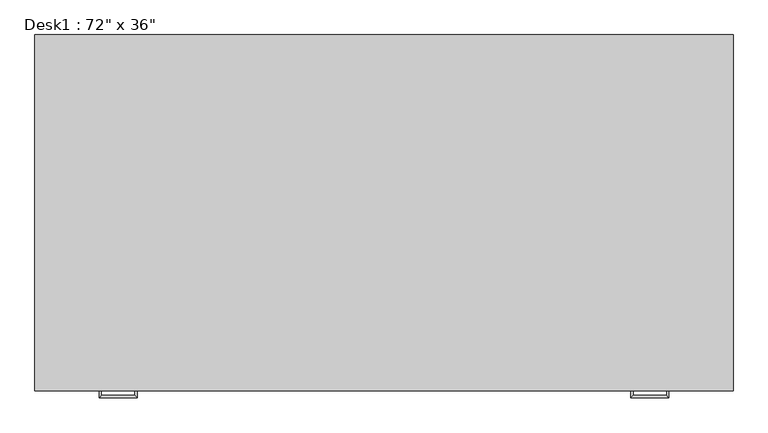
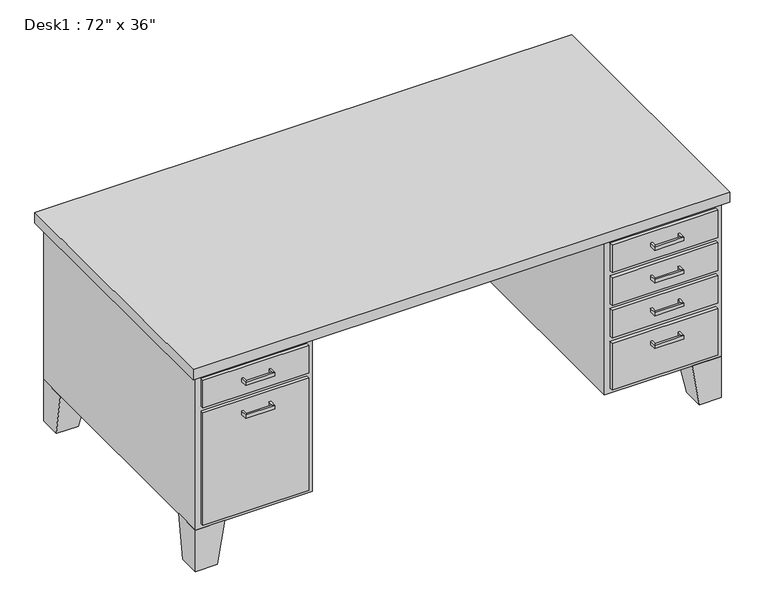
"""IFC4 building model written with IfcOpenShell, lengths in millimetres: furniture geometry."""

from ifc_helpers import new_model, si_unit, frame, origin, place, context, project, spatial, polyline, outline, extrude, faceted_brep, source, transform, mapped, element, save


def furniture_95783df2(model_context):
    return source(origin(), model_context, "Body", "SolidModel", [
        extrude(outline(polyline([(-133.35, -76.2), (234.95, -76.2), (234.95, -88.9), (-133.35, -88.9), (-133.35, -76.2)])), frame((0.0, 0.0, 603.25), z_axis=(0.0, 0.0, 1.0), x_axis=(1.0, 0.0, 0.0)), (0.0, 0.0, 1.0), 101.6),
        extrude(outline(polyline([(-133.35, -76.2), (234.95, -76.2), (234.95, -88.9), (-133.35, -88.9), (-133.35, -76.2)])), frame((0.0, 0.0, 171.45), z_axis=(0.0, 0.0, 1.0), x_axis=(1.0, 0.0, 0.0)), (0.0, 0.0, 1.0), 412.75),
        extrude(outline(polyline([(1289.05, -76.2), (1657.35, -76.2), (1657.35, -88.9), (1289.05, -88.9), (1289.05, -76.2)])), frame((0.0, 0.0, 603.25), z_axis=(0.0, 0.0, 1.0), x_axis=(1.0, 0.0, 0.0)), (0.0, 0.0, 1.0), 101.6),
        extrude(outline(polyline([(1289.05, -76.2), (1657.35, -76.2), (1657.35, -88.9), (1289.05, -88.9), (1289.05, -76.2)])), frame((0.0, 0.0, 171.45), z_axis=(0.0, 0.0, 1.0), x_axis=(1.0, 0.0, 0.0)), (0.0, 0.0, 1.0), 171.45),
        extrude(outline(polyline([(1289.05, -76.2), (1657.35, -76.2), (1657.35, -88.9), (1289.05, -88.9), (1289.05, -76.2)])), frame((0.0, 0.0, 482.6), z_axis=(0.0, 0.0, 1.0), x_axis=(1.0, 0.0, 0.0)), (0.0, 0.0, 1.0), 101.6),
        extrude(outline(polyline([(1289.05, -76.2), (1657.35, -76.2), (1657.35, -88.9), (1289.05, -88.9), (1289.05, -76.2)])), frame((0.0, 0.0, 361.95), z_axis=(0.0, 0.0, 1.0), x_axis=(1.0, 0.0, 0.0)), (0.0, 0.0, 1.0), 101.6),
        faceted_brep([(-50.8, -76.2, 152.4), (-50.8, 25.4, 152.4), (-152.4, 25.4, 152.4), (-152.4, -76.2, 152.4), (-76.2, -76.2, 0.0), (-152.4, -76.2, 0.0), (-152.4, 0.0, 0.0), (-76.2, 0.0, 0.0)], [[[0, 1, 2, 3]], [[4, 5, 6, 7]], [[4, 7, 1, 0]], [[7, 6, 2, 1]], [[6, 5, 3, 2]], [[5, 4, 0, 3]]]),
        faceted_brep([(-50.8, 838.2, 152.4), (-152.4, 838.2, 152.4), (-152.4, 736.6, 152.4), (-50.8, 736.6, 152.4), (-76.2, 838.2, 0.0), (-76.2, 762.0, 0.0), (-152.4, 762.0, 0.0), (-152.4, 838.2, 0.0)], [[[0, 1, 2, 3]], [[4, 5, 6, 7]], [[4, 7, 1, 0]], [[7, 6, 2, 1]], [[6, 5, 3, 2]], [[5, 4, 0, 3]]]),
        faceted_brep([(1574.8, 838.2, 152.4), (1574.8, 736.6, 152.4), (1676.4, 736.6, 152.4), (1676.4, 838.2, 152.4), (1600.2, 838.2, 0.0), (1676.4, 838.2, 0.0), (1676.4, 762.0, 0.0), (1600.2, 762.0, 0.0)], [[[0, 1, 2, 3]], [[4, 5, 6, 7]], [[4, 7, 1, 0]], [[7, 6, 2, 1]], [[6, 5, 3, 2]], [[5, 4, 0, 3]]]),
        faceted_brep([(1574.8, -76.2, 152.4), (1676.4, -76.2, 152.4), (1676.4, 25.4, 152.4), (1574.8, 25.4, 152.4), (1600.2, -76.2, 0.0), (1600.2, 0.0, 0.0), (1676.4, 0.0, 0.0), (1676.4, -76.2, 0.0)], [[[0, 1, 2, 3]], [[4, 5, 6, 7]], [[4, 7, 1, 0]], [[7, 6, 2, 1]], [[6, 5, 3, 2]], [[5, 4, 0, 3]]]),
        extrude(outline(polyline([(-171.45, -95.25), (-171.45, 857.25), (1695.45, 857.25), (1695.45, -95.25), (-171.45, -95.25)])), frame((0.0, 0.0, 723.9), z_axis=(0.0, 0.0, 1.0), x_axis=(1.0, 0.0, 0.0)), (0.0, 0.0, 1.0), 38.1),
        extrude(outline(polyline([(1270.0, -76.2), (1270.0, 711.2), (254.0, 711.2), (254.0, -76.2), (-152.4, -76.2), (-152.4, 838.2), (1676.4, 838.2), (1676.4, -76.2), (1270.0, -76.2)])), frame((0.0, 0.0, 152.4), z_axis=(0.0, 0.0, 1.0), x_axis=(1.0, 0.0, 0.0)), (0.0, 0.0, 1.0), 571.5),
        faceted_brep([(6.35, -88.9, 546.1), (6.35, -88.9, 533.4), (0.0, -88.9, 533.4), (0.0, -88.9, 546.1), (6.35, -107.95, 546.1), (6.35, -107.95, 533.4), (0.0, -114.3, 533.4), (0.0, -114.3, 546.1), (95.25, -107.95, 546.1), (95.25, -107.95, 533.4), (101.6, -114.3, 533.4), (101.6, -114.3, 546.1), (95.25, -88.9, 546.1), (101.6, -88.9, 546.1), (101.6, -88.9, 533.4), (95.25, -88.9, 533.4)], [[[0, 1, 2, 3]], [[1, 0, 4, 5]], [[2, 1, 5, 6]], [[3, 2, 6, 7]], [[0, 3, 7, 4]], [[5, 4, 8, 9]], [[6, 5, 9, 10]], [[7, 6, 10, 11]], [[4, 7, 11, 8]], [[12, 13, 14, 15]], [[9, 8, 12, 15]], [[10, 9, 15, 14]], [[11, 10, 14, 13]], [[8, 11, 13, 12]]]),
        faceted_brep([(6.35, -88.9, 666.75), (6.35, -88.9, 654.05), (0.0, -88.9, 654.05), (0.0, -88.9, 666.75), (6.35, -107.95, 666.75), (6.35, -107.95, 654.05), (0.0, -114.3, 654.05), (0.0, -114.3, 666.75), (95.25, -107.95, 666.75), (95.25, -107.95, 654.05), (101.6, -114.3, 654.05), (101.6, -114.3, 666.75), (95.25, -88.9, 666.75), (101.6, -88.9, 666.75), (101.6, -88.9, 654.05), (95.25, -88.9, 654.05)], [[[0, 1, 2, 3]], [[1, 0, 4, 5]], [[2, 1, 5, 6]], [[3, 2, 6, 7]], [[0, 3, 7, 4]], [[5, 4, 8, 9]], [[6, 5, 9, 10]], [[7, 6, 10, 11]], [[4, 7, 11, 8]], [[12, 13, 14, 15]], [[9, 8, 12, 15]], [[10, 9, 15, 14]], [[11, 10, 14, 13]], [[8, 11, 13, 12]]]),
        faceted_brep([(1517.65, -88.9, 304.8), (1524.0, -88.9, 304.8), (1524.0, -88.9, 292.1), (1517.65, -88.9, 292.1), (1517.65, -107.95, 304.8), (1524.0, -114.3, 304.8), (1524.0, -114.3, 292.1), (1517.65, -107.95, 292.1), (1428.75, -107.95, 304.8), (1422.4, -114.3, 304.8), (1422.4, -114.3, 292.1), (1428.75, -107.95, 292.1), (1428.75, -88.9, 304.8), (1428.75, -88.9, 292.1), (1422.4, -88.9, 292.1), (1422.4, -88.9, 304.8)], [[[0, 1, 2, 3]], [[1, 0, 4, 5]], [[2, 1, 5, 6]], [[3, 2, 6, 7]], [[0, 3, 7, 4]], [[5, 4, 8, 9]], [[6, 5, 9, 10]], [[7, 6, 10, 11]], [[4, 7, 11, 8]], [[12, 13, 14, 15]], [[9, 8, 12, 15]], [[10, 9, 15, 14]], [[11, 10, 14, 13]], [[8, 11, 13, 12]]]),
        faceted_brep([(1517.65, -88.9, 425.45), (1524.0, -88.9, 425.45), (1524.0, -88.9, 412.75), (1517.65, -88.9, 412.75), (1517.65, -107.95, 425.45), (1524.0, -114.3, 425.45), (1524.0, -114.3, 412.75), (1517.65, -107.95, 412.75), (1428.75, -107.95, 425.45), (1422.4, -114.3, 425.45), (1422.4, -114.3, 412.75), (1428.75, -107.95, 412.75), (1428.75, -88.9, 425.45), (1428.75, -88.9, 412.75), (1422.4, -88.9, 412.75), (1422.4, -88.9, 425.45)], [[[0, 1, 2, 3]], [[1, 0, 4, 5]], [[2, 1, 5, 6]], [[3, 2, 6, 7]], [[0, 3, 7, 4]], [[5, 4, 8, 9]], [[6, 5, 9, 10]], [[7, 6, 10, 11]], [[4, 7, 11, 8]], [[12, 13, 14, 15]], [[9, 8, 12, 15]], [[10, 9, 15, 14]], [[11, 10, 14, 13]], [[8, 11, 13, 12]]]),
        faceted_brep([(1517.65, -88.9, 546.1), (1524.0, -88.9, 546.1), (1524.0, -88.9, 533.4), (1517.65, -88.9, 533.4), (1517.65, -107.95, 546.1), (1524.0, -114.3, 546.1), (1524.0, -114.3, 533.4), (1517.65, -107.95, 533.4), (1428.75, -107.95, 546.1), (1422.4, -114.3, 546.1), (1422.4, -114.3, 533.4), (1428.75, -107.95, 533.4), (1428.75, -88.9, 546.1), (1428.75, -88.9, 533.4), (1422.4, -88.9, 533.4), (1422.4, -88.9, 546.1)], [[[0, 1, 2, 3]], [[1, 0, 4, 5]], [[2, 1, 5, 6]], [[3, 2, 6, 7]], [[0, 3, 7, 4]], [[5, 4, 8, 9]], [[6, 5, 9, 10]], [[7, 6, 10, 11]], [[4, 7, 11, 8]], [[12, 13, 14, 15]], [[9, 8, 12, 15]], [[10, 9, 15, 14]], [[11, 10, 14, 13]], [[8, 11, 13, 12]]]),
        faceted_brep([(1517.65, -88.9, 666.75), (1524.0, -88.9, 666.75), (1524.0, -88.9, 654.05), (1517.65, -88.9, 654.05), (1517.65, -107.95, 666.75), (1524.0, -114.3, 666.75), (1524.0, -114.3, 654.05), (1517.65, -107.95, 654.05), (1428.75, -107.95, 666.75), (1422.4, -114.3, 666.75), (1422.4, -114.3, 654.05), (1428.75, -107.95, 654.05), (1428.75, -88.9, 666.75), (1428.75, -88.9, 654.05), (1422.4, -88.9, 654.05), (1422.4, -88.9, 666.75)], [[[0, 1, 2, 3]], [[1, 0, 4, 5]], [[2, 1, 5, 6]], [[3, 2, 6, 7]], [[0, 3, 7, 4]], [[5, 4, 8, 9]], [[6, 5, 9, 10]], [[7, 6, 10, 11]], [[4, 7, 11, 8]], [[12, 13, 14, 15]], [[9, 8, 12, 15]], [[10, 9, 15, 14]], [[11, 10, 14, 13]], [[8, 11, 13, 12]]]),
    ])


if __name__ == "__main__":
    model = new_model("IFC4")
    model_context = context("Model", 3, world=origin())
    ifc_project = project(units=[si_unit("LENGTHUNIT", "METRE", prefix="MILLI")], contexts=[model_context])
    site = spatial("IfcSite", under=ifc_project)
    building = spatial("IfcBuilding", under=site)
    placement = place(None, origin())
    furniture_shape = furniture_95783df2(model_context)
    element("IfcFurniture", 1, ObjectType="Desk1 : 72\" x 36\"", at=placement, inside=building, context=model_context, shape_type="MappedRepresentation", body=[
        mapped(furniture_shape, transform((0.0, 0.0, 0.0), x_axis=(1.0, 0.0, 0.0), y_axis=(0.0, 1.0, 0.0), z_axis=(0.0, 0.0, 1.0))),
    ])
    save(model, "model.ifc")

# Revit data of these elements
# Type "Desk1 : 72\" x 36\""
#   Assembly Code = "E2020200"
#   Depth = 3' - 0"
#   Height = 2' - 6"
#   Leg Height = 0' - 6"
#   Width = 6' - 0"
#   Body Material = Laminate, Ivory, Matte
#   Handle/Leg Material = Steel, Chrome Plated
#   Top Material = Cherry
#   Default Elevation = 0
# Element 1 (IfcFurniture, "Desk1 : 72\" x 36\"")
#   Materials on its faces: "Steel, Chrome Plated", "Laminate, Ivory, Matte", "Cherry"
# Materials
#   "Laminate, Ivory, Matte": class "Plastic", colour RGB 247 247 239, transparency 0, Description = "Plastic Laminate - Ivory, Matte", Cost = 0
#   "Steel, Chrome Plated": class "Metal", colour RGB 17 17 17, transparency 0, Description = "Chromiuim plated steel", Cost = 0
#   "Cherry": class "Wood", colour RGB 226 177 128, transparency 0, Description = "Prunus Serotina", Cost = 0
